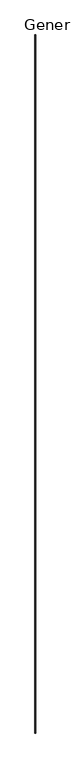
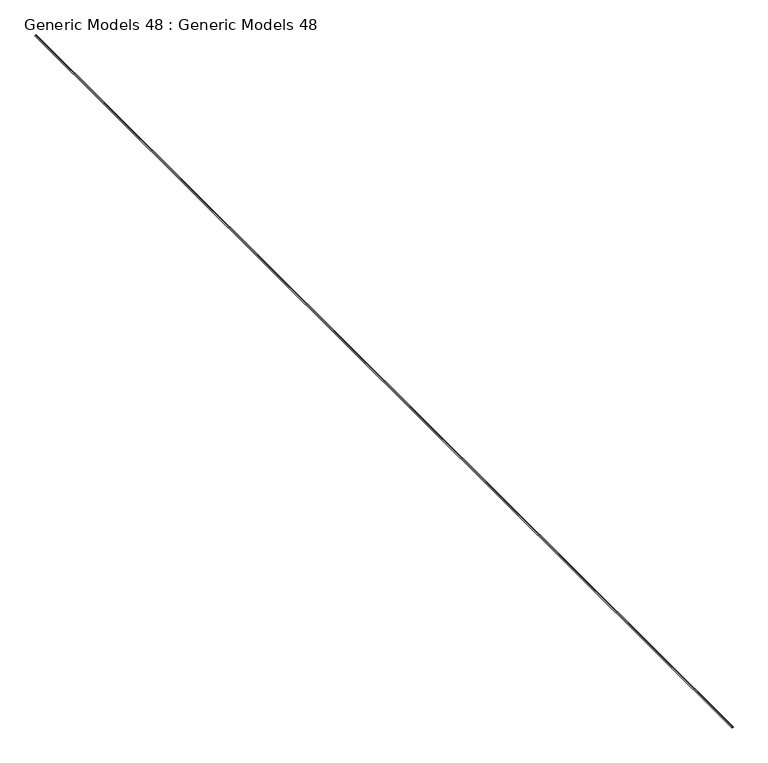
"""IFC4 building model written with IfcOpenShell, lengths in millimetres: proxy geometry, Generic Models 48 : Generic Models 48."""

import ifcopenshell
import ifcopenshell.guid

model = None  # the IFC model being written
_history = None  # IfcOwnerHistory: only IFC2X3 demands one
_inside = {}  # id of a spatial element -> (the spatial element, [elements in it])
_under = {}  # id of a project, library or spatial element -> (it, [spatial elements below it])
_declared = {}  # id of a project -> (the project, [libraries it declares])
_typed = {}  # id of a type object -> (the type object, [elements of that type])
_made_of = {}  # id of a material, layer set ... -> (it, [elements and type objects made of it])


def new_model(schema):
    """Start an empty IFC model of exactly this schema.

    Asked for "IFC4X3", IfcOpenShell would pick the latest addendum, in which some entities
    have other attributes; the version numbers below select the first issue.
    IFC2X3 requires an IfcOwnerHistory on every rooted entity: one is made here for all.
    """
    global model, _history
    if schema == "IFC4X3":
        model = ifcopenshell.file(schema_version=(4, 3, 0, 0))
    else:
        model = ifcopenshell.file(schema=schema)
    _inside.clear()
    _under.clear()
    _declared.clear()
    _typed.clear()
    _made_of.clear()
    _history = None
    if model.schema == "IFC2X3":
        org = make("IfcOrganization", Name="unknown")
        user = make(
            "IfcPersonAndOrganization",
            ThePerson=make("IfcPerson", FamilyName="unknown"),
            TheOrganization=org,
        )
        app = make(
            "IfcApplication",
            ApplicationDeveloper=org,
            Version="unknown",
            ApplicationFullName="unknown",
            ApplicationIdentifier="unknown",
        )
        _history = make(
            "IfcOwnerHistory",
            OwningUser=user,
            OwningApplication=app,
            ChangeAction="ADDED",
            CreationDate=0,
        )
    return model


def make(cls, **values):
    """One entity of the class cls with the attributes given. An attribute that is None is left unset."""
    return model.create_entity(
        cls, **{name: value for name, value in values.items() if value is not None}
    )


def rooted(cls, **values):
    """An entity with a GlobalId (a new one), such as an element, a storey or a relation."""
    return make(cls, GlobalId=ifcopenshell.guid.new(), OwnerHistory=_history, **values)


def si_unit(unit_type, name, prefix=None):
    """IfcSIUnit, for example si_unit("LENGTHUNIT", "METRE", prefix="MILLI")."""
    return make("IfcSIUnit", UnitType=unit_type, Prefix=prefix, Name=name)


def assignment(units):
    """IfcUnitAssignment: the units of a project."""
    return None if units is None else make("IfcUnitAssignment", Units=units)


def point(xyz):
    """IfcCartesianPoint."""
    return None if xyz is None else make("IfcCartesianPoint", Coordinates=xyz)


def direction(xyz):
    """IfcDirection."""
    return None if xyz is None else make("IfcDirection", DirectionRatios=xyz)


def frame(location, z_axis=None, x_axis=None):
    """IfcAxis2Placement3D, a coordinate frame: its origin and axes. An axis left out is left unset."""
    return make(
        "IfcAxis2Placement3D",
        Location=point(location),
        Axis=direction(z_axis),
        RefDirection=direction(x_axis),
    )


def origin():
    """The frame at (0, 0, 0) with its axes left unset."""
    return frame((0.0, 0.0, 0.0))


def place(relative_to, where):
    """IfcLocalPlacement: puts the frame where relative to a parent placement (None: the world)."""
    return make(
        "IfcLocalPlacement", PlacementRelTo=relative_to, RelativePlacement=where
    )


def context(
    kind, dimensions, precision=None, world=None, true_north=None, identifier=None
):
    """IfcGeometricRepresentationContext, for example the 3D "Model" context."""
    return make(
        "IfcGeometricRepresentationContext",
        ContextIdentifier=identifier,
        ContextType=kind,
        CoordinateSpaceDimension=dimensions,
        Precision=precision,
        WorldCoordinateSystem=world,
        TrueNorth=true_north,
    )


def project(units=None, contexts=None):
    """IfcProject with its units and contexts."""
    return rooted(
        "IfcProject",
        Name="project",
        RepresentationContexts=contexts,
        UnitsInContext=assignment(units),
    )


def spatial(cls, under=None, at=None, **own):
    """A site, building, storey or space (cls), placed at a placement, below another one or the project."""
    s = rooted(cls, ObjectPlacement=at, **own)
    if under is not None:
        _under.setdefault(under.id(), (under, []))[1].append(s)
    return s


def polyline(points):
    """IfcPolyline through the points."""
    return make("IfcPolyline", Points=[point(p) for p in points])


def circle_curve(where, radius):
    """IfcCircle in the frame where."""
    return make("IfcCircle", Position=where, Radius=radius)


def ellipse_curve(where, semi_axis1, semi_axis2):
    """IfcEllipse in the frame where."""
    return make(
        "IfcEllipse", Position=where, SemiAxis1=semi_axis1, SemiAxis2=semi_axis2
    )


def trimmed(basis, trim1, trim2, sense, master):
    """IfcTrimmedCurve: the piece of a basis curve between two trims."""
    return make(
        "IfcTrimmedCurve",
        BasisCurve=basis,
        Trim1=trim1,
        Trim2=trim2,
        SenseAgreement=sense,
        MasterRepresentation=master,
    )


def shape(context_of_items, identifier, shape_type, items):
    """IfcShapeRepresentation: the items that make up one representation, for example the "Body"."""
    return make(
        "IfcShapeRepresentation",
        ContextOfItems=context_of_items,
        RepresentationIdentifier=identifier,
        RepresentationType=shape_type,
        Items=items,
    )


def source(mapping_origin, context_of_items, identifier, shape_type, items):
    """IfcRepresentationMap: a shape defined once, which mapped items show again and again."""
    return make(
        "IfcRepresentationMap",
        MappingOrigin=mapping_origin,
        MappedRepresentation=shape(context_of_items, identifier, shape_type, items),
    )


def transform(
    local_origin,
    x_axis=None,
    y_axis=None,
    z_axis=None,
    scale=None,
    scale2=None,
    scale3=None,
    uniform=True,
):
    """IfcCartesianTransformationOperator3D, or its non-uniform kind. x_axis, y_axis, z_axis: its Axis1, 2, 3."""
    if uniform:
        return make(
            "IfcCartesianTransformationOperator3D",
            Axis1=direction(x_axis),
            Axis2=direction(y_axis),
            LocalOrigin=point(local_origin),
            Scale=scale,
            Axis3=direction(z_axis),
        )
    return make(
        "IfcCartesianTransformationOperator3DnonUniform",
        Axis1=direction(x_axis),
        Axis2=direction(y_axis),
        LocalOrigin=point(local_origin),
        Scale=scale,
        Axis3=direction(z_axis),
        Scale2=scale2,
        Scale3=scale3,
    )


def mapped(mapping_source, mapping_target):
    """IfcMappedItem: shows the shape of a source again, moved by a transform."""
    return make(
        "IfcMappedItem", MappingSource=mapping_source, MappingTarget=mapping_target
    )


def made_of(thing, what):
    """Note that an element or type object is made of a material, layer set ...; save() writes the relation."""
    if what is not None:
        _made_of.setdefault(what.id(), (what, []))[1].append(thing)
    return thing


def element(
    cls,
    number,
    at=None,
    inside=None,
    cuts=None,
    type_object=None,
    material=None,
    context=None,
    identifier="Body",
    shape_type=None,
    held_by="IfcProductDefinitionShape",
    body=None,
    shapes=None,
    **own,
):
    """One element of the class cls, such as IfcWall. Its Tag is "e" and its number.

    at: its placement. inside: the storey or other place that contains it. cuts: it is an
    opening in that element (IfcRelVoidsElement). A single representation is given by context,
    identifier, shape_type and body (its items); several are given by shapes. held_by: the class
    of the entity that holds the representations. save() writes the other relations.
    """
    e = rooted(cls, Tag="e%d" % number, ObjectPlacement=at, **own)
    if body is not None:
        shapes = [shape(context, identifier, shape_type, body)]
    if shapes is not None:
        e.Representation = make(held_by, Representations=shapes)
    if inside is not None:
        _inside.setdefault(inside.id(), (inside, []))[1].append(e)
    if cuts is not None:
        rooted(
            "IfcRelVoidsElement", RelatingBuildingElement=cuts, RelatedOpeningElement=e
        )
    if type_object is not None:
        _typed.setdefault(type_object.id(), (type_object, []))[1].append(e)
    return made_of(e, material)


def aggregate(whole, parts):
    """IfcRelAggregates: a whole, such as a stair, and the parts it consists of."""
    return rooted("IfcRelAggregates", RelatingObject=whole, RelatedObjects=parts)


def save(model, path):
    """Write the relations noted so far, then the file.

    IfcRelAggregates (storeys below a building ...), IfcRelContainedInSpatialStructure (elements
    in a storey), IfcRelDefinesByType, IfcRelAssociatesMaterial and IfcRelDeclares: one each for
    every whole, place, type object, material and project.
    """
    for whole, parts in _under.values():
        aggregate(whole, parts)
    for where, things in _inside.values():
        rooted(
            "IfcRelContainedInSpatialStructure",
            RelatedElements=things,
            RelatingStructure=where,
        )
    for kind, things in _typed.values():
        rooted("IfcRelDefinesByType", RelatedObjects=things, RelatingType=kind)
    for what, things in _made_of.values():
        rooted("IfcRelAssociatesMaterial", RelatedObjects=things, RelatingMaterial=what)
    for by, libraries in _declared.values():
        rooted("IfcRelDeclares", RelatingContext=by, RelatedDefinitions=libraries)
    model.write(path)


def plane_surface(at):
    """IfcPlane: the flat surface through the origin of the frame at, square to its z axis."""
    return make("IfcPlane", Position=at)


def cylinder_surface(at, radius):
    """IfcCylindricalSurface: all points at the distance radius from the z axis of the frame at."""
    return make("IfcCylindricalSurface", Position=at, Radius=radius)


def revolved_surface(curve, axis_point, axis_direction):
    """IfcSurfaceOfRevolution: the curve turned about the line through axis_point along axis_direction."""
    return make(
        "IfcSurfaceOfRevolution",
        SweptCurve=make("IfcArbitraryOpenProfileDef", ProfileType="CURVE", Curve=curve),
        AxisPosition=make("IfcAxis1Placement", Location=point(axis_point), Axis=direction(axis_direction)),
    )


def extruded_surface(curve, direction_of_extrusion, depth):
    """IfcSurfaceOfLinearExtrusion: the curve pushed along a direction by depth."""
    return make(
        "IfcSurfaceOfLinearExtrusion",
        SweptCurve=make("IfcArbitraryOpenProfileDef", ProfileType="CURVE", Curve=curve),
        ExtrudedDirection=direction(direction_of_extrusion),
        Depth=depth,
    )


def advanced_brep(points, edges, surfaces, faces):
    """IfcAdvancedBrep: a solid bounded by faces that lie on surfaces and meet in shared edges.

    An edge is (start, end): straight between two places in points (the first is 0);
    or (start, end, curve); or (start, end, curve, False) where it runs against its curve.
    A face is (place in surfaces, loops), or (place, loops, False) where it looks against
    its surface's normal. A loop lists edges by number (the first is 1), with a minus sign
    where the edge is run from its end to its start. The first loop is the outer one.
    """
    corners = [point(p) for p in points]
    vertices = [make("IfcVertexPoint", VertexGeometry=c) for c in corners]
    made = []
    for start, end, *more in edges:
        made.append(
            make(
                "IfcEdgeCurve",
                EdgeStart=vertices[start],
                EdgeEnd=vertices[end],
                EdgeGeometry=more[0] if more else make("IfcPolyline", Points=[corners[start], corners[end]]),
                SameSense=more[1] if len(more) > 1 else True,
            )
        )
    hull = []
    for where, loops, *sense in faces:
        bounds = []
        for j, loop in enumerate(loops):
            ring = [make("IfcOrientedEdge", EdgeElement=made[abs(k) - 1], Orientation=k > 0) for k in loop]
            bounds.append(
                make(
                    "IfcFaceOuterBound" if j == 0 else "IfcFaceBound",
                    Bound=make("IfcEdgeLoop", EdgeList=ring),
                    Orientation=True,
                )
            )
        hull.append(make("IfcAdvancedFace", Bounds=bounds, FaceSurface=surfaces[where], SameSense=sense[0] if sense else True))
    return make("IfcAdvancedBrep", Outer=make("IfcClosedShell", CfsFaces=hull))


def generic_models_48_generic_models_48_07923f71(model_context):
    return source(origin(), model_context, "Body", "AdvancedBrep", [
        advanced_brep(
        [(32143.0590778, 29574.9917286, 269371.1566688), (32139.8840778, 29574.9917286, 269371.1566688), (32138.9323185, 29574.9917286, 269369.8860102), (32138.9323185, 29574.9917286, 269366.0773273), (32139.8840778, 29574.9917286, 269364.8066688), (32143.0590778, 29574.9917286, 269364.8066688), (32143.0590778, 40781.6231612, 269371.1566688), (32143.0590778, 40781.6231612, 269364.8066688), (32139.8840778, 40781.6231612, 269364.8066688), (32138.9323185, 40781.6231612, 269366.0773273), (32138.9323185, 40781.6231612, 269369.8860102), (32139.8840778, 40781.6231612, 269371.1566688)],
        [
            (0, 1),
            (1, 2, circle_curve(frame((32142.7988183, 29574.9917286, 269367.9816688), z_axis=(0.0, -1.0, 0.0), x_axis=(0.0, 0.0, 1.0)), 4.3100275)),
            (2, 3, ellipse_curve(frame((32135.1215778, 29574.9917286, 269367.9816688), z_axis=(0.0, -1.0, 0.0), x_axis=(1.0, 0.0, 0.0)), 4.7625, 3.175)),
            (3, 4, circle_curve(frame((32142.7988183, 29574.9917286, 269367.9816688), z_axis=(0.0, -1.0, 0.0), x_axis=(0.0, 0.0, 1.0)), 4.3100275)),
            (4, 5),
            (5, 0, circle_curve(frame((32145.9738183, 29574.9917286, 269367.9816688), z_axis=(0.0, 1.0, 0.0), x_axis=(0.0, 0.0, 1.0)), 4.3100275)),
            (6, 7, circle_curve(frame((32145.9738183, 40781.6231612, 269367.9816688), z_axis=(0.0, -1.0, 0.0), x_axis=(0.0, 0.0, 1.0)), 4.3100275)),
            (7, 8),
            (8, 9, circle_curve(frame((32142.7988183, 40781.6231612, 269367.9816688), z_axis=(0.0, 1.0, 0.0), x_axis=(0.0, 0.0, 1.0)), 4.3100275)),
            (9, 10, ellipse_curve(frame((32135.1215778, 40781.6231612, 269367.9816688), z_axis=(0.0, 1.0, 0.0), x_axis=(1.0, 0.0, 0.0)), 4.7625, 3.175)),
            (10, 11, circle_curve(frame((32142.7988183, 40781.6231612, 269367.9816688), z_axis=(0.0, 1.0, 0.0), x_axis=(0.0, 0.0, 1.0)), 4.3100275)),
            (11, 6),
            (0, 6),
            (11, 1),
            (10, 2),
            (9, 3),
            (8, 4),
            (7, 5),
        ],
        [
            plane_surface(frame((32143.0590778, 29574.9917286, 269364.8066688), z_axis=(0.0, -1.0, 0.0), x_axis=(1.0, 0.0, 0.0))),
            plane_surface(frame((32143.0590778, 40781.6231612, 269364.8066688), z_axis=(0.0, 1.0, 0.0), x_axis=(1.0, 0.0, 0.0))),
            plane_surface(frame((32143.0590778, 29574.9917286, 269371.1566688), z_axis=(0.0, 0.0, 1.0), x_axis=(0.0, 1.0, 0.0))),
            cylinder_surface(frame((32142.7988183, 29574.9917286, 269367.9816688), z_axis=(0.0, -1.0, 0.0), x_axis=(0.0, 0.0, 1.0)), 4.3100275),
            extruded_surface(trimmed(ellipse_curve(frame((32135.1215778, 40781.6231612, 269367.9816688), z_axis=(0.0, -1.0, 0.0), x_axis=(1.0, 0.0, 0.0)), 4.7625, 3.175), [point((32138.9323185, 40781.6231612, 269369.8860102))], [point((32138.9323185, 40781.6231612, 269366.0773273))], True, "CARTESIAN"), (0.0, -11206.631432599996, 0.0), 11206.631432599996),
            plane_surface(frame((32139.8840778, 29574.9917286, 269364.8066688), z_axis=(0.0, 0.0, -1.0), x_axis=(0.0, 1.0, 0.0))),
            revolved_surface(polyline([(32145.9738183, 40781.6231612, 269372.2916963), (32145.9738183, 29574.9917286, 269372.2916963)]), (32145.9738183, 29574.9917286, 269367.9816688), (0.0, 1.0, 0.0)),
        ],
        [
            (0, [[1, 2, 3, 4, 5, 6]]),
            (1, [[7, 8, 9, 10, 11, 12]]),
            (2, [[-1, 13, -12, 14]]),
            (3, [[-2, -14, -11, 15]]),
            (4, [[-3, -15, -10, 16]]),
            (3, [[-4, -16, -9, 17]]),
            (5, [[-5, -17, -8, 18]]),
            (6, [[-6, -18, -7, -13]]),
        ],
    ),
    ])


if __name__ == "__main__":
    model = new_model("IFC4")
    model_context = context("Model", 3, world=origin())
    ifc_project = project(units=[si_unit("LENGTHUNIT", "METRE", prefix="MILLI")], contexts=[model_context])
    site = spatial("IfcSite", under=ifc_project)
    building = spatial("IfcBuilding", under=site)
    placement = place(None, origin())
    generic_models_48_generic_models_48_shape = generic_models_48_generic_models_48_07923f71(model_context)
    element("IfcBuildingElementProxy", 1, Name="Generic Models 48 : Generic Models 48", ObjectType="Generic Models 48 : Generic Models 48", at=placement, inside=building, context=model_context, shape_type="MappedRepresentation", body=[
        mapped(generic_models_48_generic_models_48_shape, transform((0.0, 0.0, 0.0), x_axis=(1.0, 0.0, 0.0), y_axis=(0.0, 1.0, 0.0), z_axis=(0.0, 0.0, 1.0))),
    ])
    save(model, "model.ifc")

# Revit data of these elements
# Element 1 (IfcBuildingElementProxy, "Generic Models 48 : Generic Models 48")
#   Materials on its faces: "SEALANT (& BACKER ROD IF NECESSARY)"
# Materials
#   "SEALANT (& BACKER ROD IF NECESSARY)": class "Generic", colour RGB 176 213 108, transparency 0, Cost = 0
